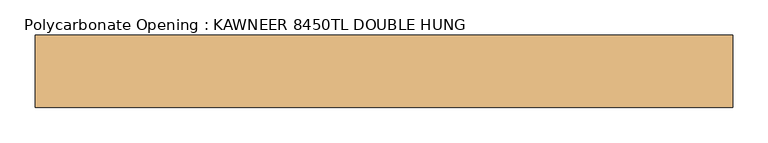
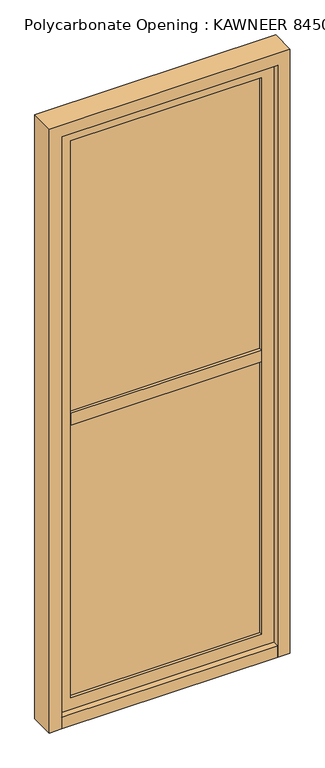
"""IFC4 building model written with IfcOpenShell, lengths in millimetres: door geometry, Polycarbonate Opening : KAWNEER 8450TL DOUBLE HUNG."""

from ifc_helpers import new_model, si_unit, frame, origin, origin_with_axes, place, context, project, spatial, polyline, outline, extrude, source, transform, mapped, element, save


def polycarbonate_opening_kawneer_8450tl_double_hung_ba695106(model_context):
    return source(origin(), model_context, "Body", "SweptSolid", [
        extrude(outline(polyline([(440.1908884, 12.7), (440.1908884, -12.7), (-440.1908884, -12.7), (-440.1908884, 12.7), (440.1908884, 12.7)])), frame((0.0, 0.0, 50.8), z_axis=(0.0, 0.0, 1.0), x_axis=(1.0, 0.0, 0.0)), (0.0, 0.0, 1.0), 2498.4648118),
        extrude(outline(polyline([(2549.2648118, -440.1908884), (0.0, -440.1908884), (0.0, 440.1908884), (2549.2648118, 440.1908884), (2549.2648118, -440.1908884)]), holes=[polyline([(101.6, 389.3908884), (101.6, -389.3908884), (2498.4648118, -389.3908884), (2498.4648118, 389.3908884), (101.6, 389.3908884)])]), frame((0.0, -25.4, 0.0), z_axis=(0.0, 1.0, 0.0), x_axis=(0.0, 0.0, 1.0)), (0.0, 0.0, 1.0), 50.8),
        extrude(outline(polyline([(2600.0648118, 490.9908884), (2600.0648118, -490.9908884), (0.0, -490.9908884), (0.0, -440.1908884), (2549.2648118, -440.1908884), (2549.2648118, 440.1908884), (0.0, 440.1908884), (0.0, 490.9908884), (2600.0648118, 490.9908884)])), frame((0.0, -50.8, 0.0), z_axis=(0.0, 1.0, 0.0), x_axis=(0.0, 0.0, 1.0)), (0.0, 0.0, 1.0), 101.6),
        extrude(outline(polyline([(389.3908884, 25.4), (389.3908884, -25.4), (-389.3908884, -25.4), (-389.3908884, 25.4), (389.3908884, 25.4)])), frame((0.0, 0.0, 1274.6324059), z_axis=(0.0, 0.0, 1.0), x_axis=(1.0, 0.0, 0.0)), (0.0, 0.0, 1.0), 50.8),
        extrude(outline(polyline([(440.1908884, 50.8), (440.1908884, -50.8), (-440.1908884, -50.8), (-440.1908884, 50.8), (440.1908884, 50.8)])), origin_with_axes(), (0.0, 0.0, 1.0), 50.8),
    ])


if __name__ == "__main__":
    model = new_model("IFC4")
    model_context = context("Model", 3, world=origin())
    ifc_project = project(units=[si_unit("LENGTHUNIT", "METRE", prefix="MILLI")], contexts=[model_context])
    site = spatial("IfcSite", under=ifc_project)
    building = spatial("IfcBuilding", under=site)
    placement = place(None, origin())
    polycarbonate_opening_kawneer_8450tl_double_hung_shape = polycarbonate_opening_kawneer_8450tl_double_hung_ba695106(model_context)
    element("IfcDoor", 1, ObjectType="Polycarbonate Opening : KAWNEER 8450TL DOUBLE HUNG", at=placement, inside=building, context=model_context, shape_type="MappedRepresentation", body=[
        mapped(polycarbonate_opening_kawneer_8450tl_double_hung_shape, transform((0.0, 0.0, 0.0), x_axis=(1.0, 0.0, 0.0), y_axis=(0.0, 1.0, 0.0), z_axis=(0.0, 0.0, 1.0))),
    ])
    save(model, "model.ifc")

# Revit data of these elements
# Type "Polycarbonate Opening : KAWNEER 8450TL DOUBLE HUNG"
#   Type Mark = "59"
#   OD_DS_Door_Material = "ALUM./GLAZING"
#   OD_DS_Door_Type = "STOREFRONT - DOUBLE HUNG WINDOW"
#   OD_DS_Lockset = "POLE OPERATOR HARDWARE FOR TOP SASH; BOTTOM SASH MECHANICALLY FIXED"
#   Analytic Construction = "<None>"
#   offset [instance default] = 0' - 2"
#   Stile = 0' - 2"
#   Mullion Width = 0' - 2"
#   Mullion Depth = 0' - 4"
#   Opening Size [instance default] = 5' - 1.50212"
#   Door Width [instance default] = 5' - 1.50212"
#   Window ON/OFF = no
#   Door On/Off = yes
#   Mullion Material = DOUBLE HUNG (CLEAR ANODIZED ALUM) - TEMPERED INSULATED GLAZING (CARDINAL GLASS LoĒ²-240\nOR EQUIVALENT)
#   Glass Material = TEMPERED INSULATED GLAZING (CARDINAL GLASS LoĒ²-240\nOR EQUIVALENT)
#   Door Material = DOUBLE HUNG (CLEAR ANODIZED ALUM) - TEMPERED INSULATED GLAZING (CARDINAL GLASS LoĒ²-240\nOR EQUIVALENT)
# Element 1 (IfcDoor, "Polycarbonate Opening : KAWNEER 8450TL DOUBLE HUNG")
#   offset = 0' - 0"
#   Materials on its faces: "DOUBLE HUNG (CLEAR ANODIZED ALUM) - TEMPERED INSULATED GLAZING (CARDINAL GLASS LoĒ²-240\nOR EQUIVALENT)", "TEMPERED INSULATED GLAZING (CARDINAL GLASS LoĒ²-240\nOR EQUIVALENT)"
# Materials
#   "DOUBLE HUNG (CLEAR ANODIZED ALUM) - TEMPERED INSULATED GLAZING (CARDINAL GLASS LoĒ²-240\nOR EQUIVALENT)": class "Metal", colour RGB 244 244 244, transparency 0, Description = "Aluminum 6061", Cost = 0
#   "TEMPERED INSULATED GLAZING (CARDINAL GLASS LoĒ²-240\nOR EQUIVALENT)": class "Glass", colour RGB 196 205 210, transparency 0.85, Description = "Soda Lime Glass", Cost = 0
